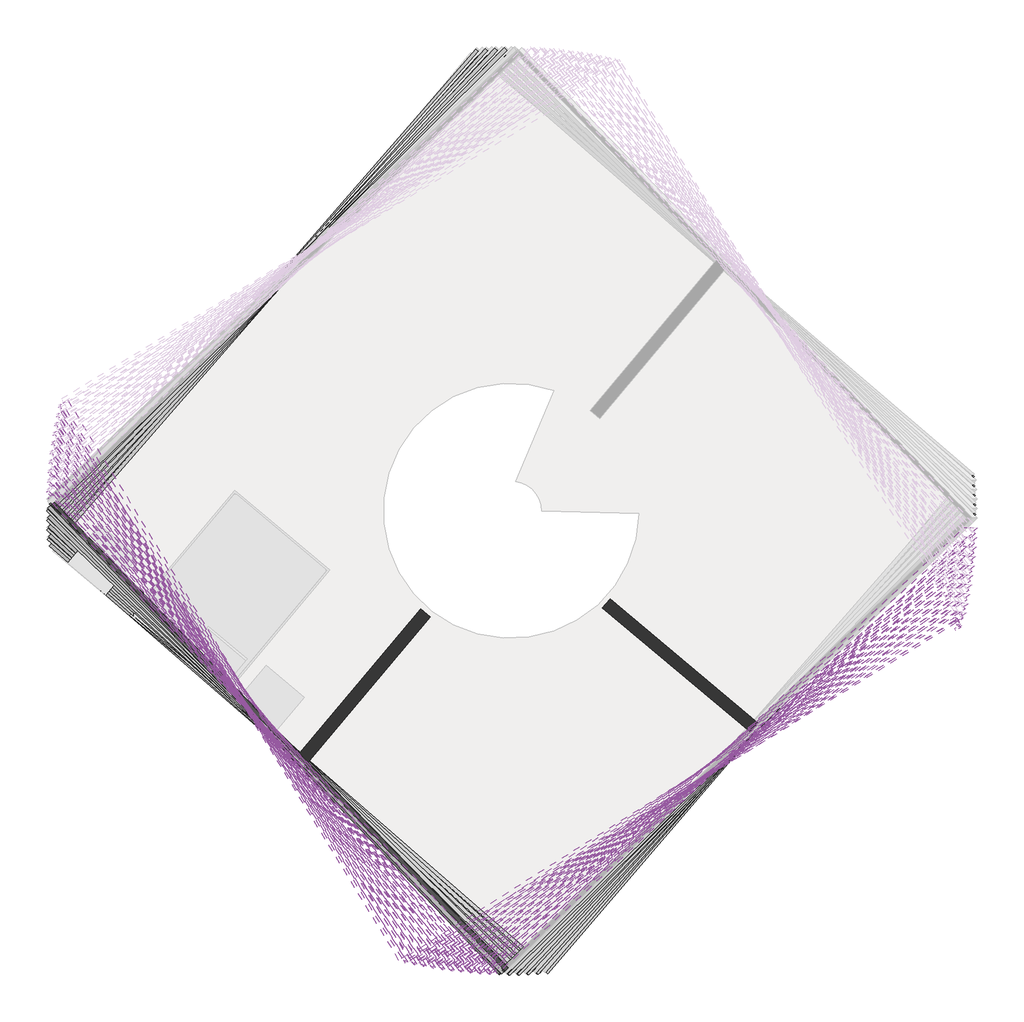
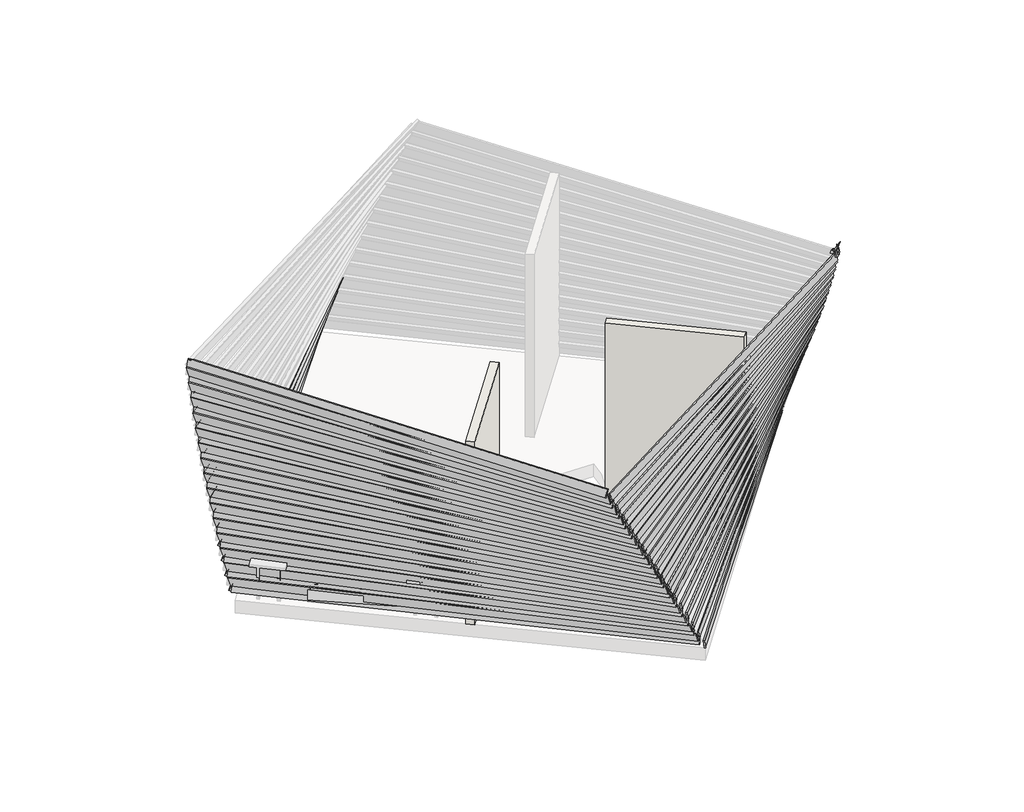
# One storey, part 1 of 2: 33 plates, 32 members, 2 walls.
# Revit data of these elements (continued)
# Project information
#   Project Issue Date = "28/5/20"
#   Project Status = "Project  Status"
#   Client Name = "Dafni Levy"
#   Project Address = "## Street\nCity, State  Zip"
#   Project Name = "In the Heights"
#   Project Number = "1"
# Type "Rectangular Mullion : tilted mullions"
#   built-in parameter 1007304 = 0.492126 (stored number, unit not read)
#   built-in parameter 1007301 = 0.082021 (stored number, unit not read)
#   built-in parameter 1007300 = 0.082021 (stored number, unit not read)
# Type "Generic - 150mm"
#   Layers, outside or top first: 0.15 m no material (function 1)
# Elements 1, 2, 3, 4, 5, 6, 7, 8, 9, 10, 11, 12, 13, 14, 15, 16, 17, 18, 19, 20, 21, 22, 23, 24, 25, 26, 27, 28, 29, 30, 31, 32 (IfcMember, "Rectangular Mullion : tilted mullions")
#   Phase Created = New Construction
#   Materials on its faces: "Aluminum"
# Elements 33, 34, 35, 36, 37, 38, 39, 40, 41, 42, 43, 44, 45, 46, 47, 48, 49, 50, 51, 52, 53, 54, 55, 56, 57, 58, 59, 60, 61, 62, 63, 64, 65 (IfcPlate, "System Panel : Glazed")
#   Phase Created = New Construction
#   Materials on its faces: "Glass"
# Elements 66, 67 (IfcWall, "Generic - 150mm")
#   Top Offset = 0.00 m
#   Base Offset = 0.00 m
#   wall height = 3.745 m
#   Phase Created = New Construction
#   Base Constraint = Planta Arquitectonica Nivel 200
#   Top Constraint = Planta Arquitectonica Nivel 300
#   Materials on its faces: "Default Wall"
# Materials
#   "Aluminum": class "Metal", colour RGB 244 244 244, transparency 0, Description = "Aluminum 6061", Cost = 0
#   "Glass": class "Glass", colour RGB 218 227 224, transparency 0.85, Description = "Soda Lime Glass", Cost = 0
#   "Default Wall": class "Miscellaneous", colour RGB 80 80 80, transparency 0
# Area, not placed, upper offset 0.00 m, lower offset 0.00 m
#   Number = "5"
#   Name = "Area"
# Area, not placed, upper offset 0.00 m, lower offset 0.00 m
#   Number = "6"
#   Name = "Area"
# Area at (2560.045, 1794.583) mm, upper offset 0.00 m, lower offset 0.00 m
#   Number = "7"
#   Name = "Dormitorio"
# Area at (2857.046, -2759.433) mm, upper offset 0.00 m, lower offset 0.00 m
#   Number = "8"
#   Name = "Oficina"
